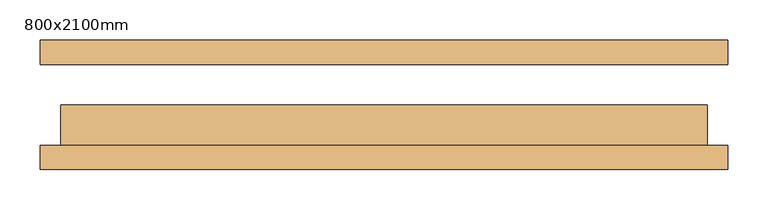
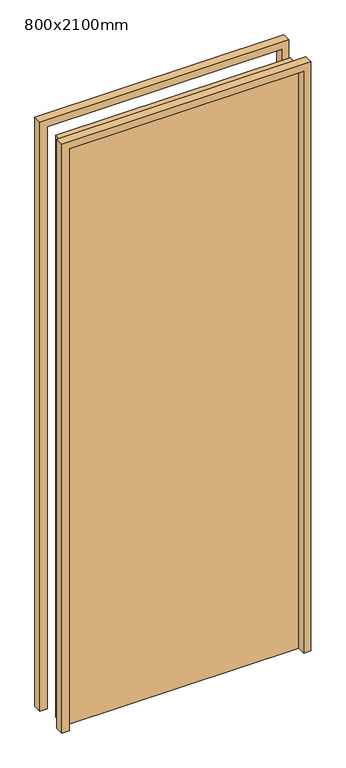
"""IFC4 building model written with IfcOpenShell, lengths in millimetres: door geometry, WWm-SingleSolid-Flush : 800x2100mm."""

from ifc_helpers import new_model, si_unit, frame, origin, origin_with_axes, place, context, project, spatial, polyline, outline, extrude, source, transform, mapped, element, save


def door_800x2100mm_760b0b47(model_context):
    return source(origin(), model_context, "Body", "SweptSolid", [
        extrude(outline(polyline([(2125.0, -425.0), (0.0, -425.0), (0.0, -400.0), (2100.0, -400.0), (2100.0, 400.0), (0.0, 400.0), (0.0, 425.0), (2125.0, 425.0), (2125.0, -425.0)])), frame((0.0, -80.0, 0.0), z_axis=(0.0, 1.0, 0.0), x_axis=(0.0, 0.0, 1.0)), (0.0, 0.0, 1.0), 30.0),
        extrude(outline(polyline([(2125.0, 425.0), (2125.0, -425.0), (0.0, -425.0), (0.0, -400.0), (2100.0, -400.0), (2100.0, 400.0), (0.0, 400.0), (0.0, 425.0), (2125.0, 425.0)])), frame((0.0, 50.0, 0.0), z_axis=(0.0, 1.0, 0.0), x_axis=(0.0, 0.0, 1.0)), (0.0, 0.0, 1.0), 30.0),
        extrude(outline(polyline([(400.0, 0.0), (400.0, -50.0), (-400.0, -50.0), (-400.0, 0.0), (400.0, 0.0)])), origin_with_axes(), (0.0, 0.0, 1.0), 2100.0),
    ])


if __name__ == "__main__":
    model = new_model("IFC4")
    model_context = context("Model", 3, world=origin())
    ifc_project = project(units=[si_unit("LENGTHUNIT", "METRE", prefix="MILLI")], contexts=[model_context])
    site = spatial("IfcSite", under=ifc_project)
    building = spatial("IfcBuilding", under=site)
    placement = place(None, origin())
    door_800x2100mm_shape = door_800x2100mm_760b0b47(model_context)
    element("IfcDoor", 1, ObjectType="WWm-SingleSolid-Flush : 800x2100mm", at=placement, inside=building, context=model_context, shape_type="MappedRepresentation", body=[
        mapped(door_800x2100mm_shape, transform((0.0, 0.0, 0.0), x_axis=(1.0, 0.0, 0.0), y_axis=(0.0, 1.0, 0.0), z_axis=(0.0, 0.0, 1.0))),
    ])
    save(model, "model.ifc")

# Revit data of these elements
# Type "WWm-SingleSolid-Flush : 800x2100mm"
#   Type Mark = "EX1-54"
#   Construction Type Id = "MDOOR"
#   Assembly Code = "C1020"
#   Analytic Construction = "Metal"
#   Thickness = 50 mm
#   Thermal Resistance (R) = 0.270117 (m²·K)/W
#   Heat Transfer Coefficient (U) = 3.7021 W/(m²·K)
#   Height = 2100 mm
#   Trim Projection Ext = 30 mm
#   Trim Projection Int = 30 mm
#   Trim Width = 25 mm
#   Width = 800 mm
#   Not 90 Degree [instance default] = no
#   90 Degree [instance default] = yes
#   Door Material = WW-EC-RGB-White
#   Frame Material = WW-EC-RGB-White
#   Visual Light Transmittance = 0
#   Solar Heat Gain Coefficient = 0
#   Function = (empty or 0)
#   Wall Closure = (empty or 0)
# Element 1 (IfcDoor, "WWm-SingleSolid-Flush : 800x2100mm")
#   Materials on its faces: "WW-EC-RGB-White"
# Materials
#   "WW-EC-RGB-White": class "Generic", colour RGB 255 255 255, transparency 0, Comments = "If region requests off-white, swith asset color to RGB 231-228-220", Description = "Generic Color", Cost = 0
